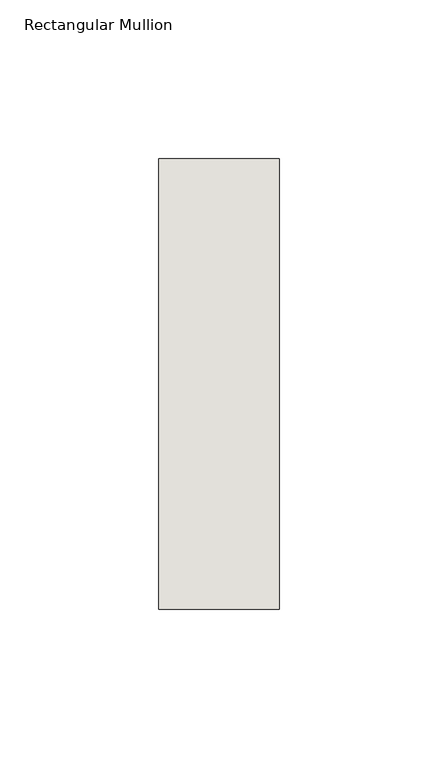
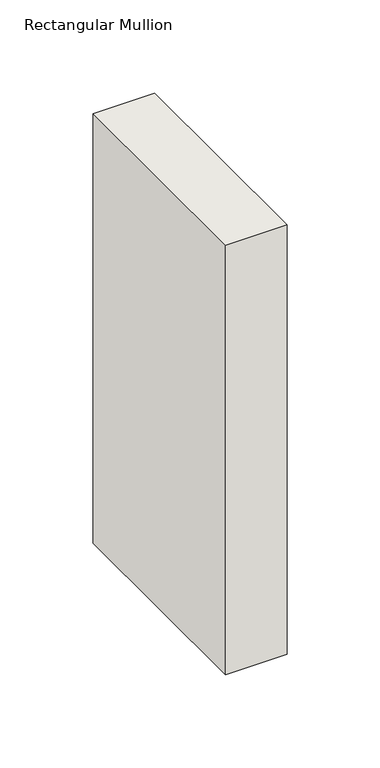
"""IFC4 building model written with IfcOpenShell, lengths in millimetres: wall geometry, Rectangular Mullion : NLRS_21_CWM_hsb-regel 38x142_gen_rsf."""

import ifcopenshell
import ifcopenshell.guid

model = None  # the IFC model being written
_history = None  # IfcOwnerHistory: only IFC2X3 demands one
_inside = {}  # id of a spatial element -> (the spatial element, [elements in it])
_under = {}  # id of a project, library or spatial element -> (it, [spatial elements below it])
_declared = {}  # id of a project -> (the project, [libraries it declares])
_typed = {}  # id of a type object -> (the type object, [elements of that type])
_made_of = {}  # id of a material, layer set ... -> (it, [elements and type objects made of it])


def new_model(schema):
    """Start an empty IFC model of exactly this schema.

    Asked for "IFC4X3", IfcOpenShell would pick the latest addendum, in which some entities
    have other attributes; the version numbers below select the first issue.
    IFC2X3 requires an IfcOwnerHistory on every rooted entity: one is made here for all.
    """
    global model, _history
    if schema == "IFC4X3":
        model = ifcopenshell.file(schema_version=(4, 3, 0, 0))
    else:
        model = ifcopenshell.file(schema=schema)
    _inside.clear()
    _under.clear()
    _declared.clear()
    _typed.clear()
    _made_of.clear()
    _history = None
    if model.schema == "IFC2X3":
        org = make("IfcOrganization", Name="unknown")
        user = make(
            "IfcPersonAndOrganization",
            ThePerson=make("IfcPerson", FamilyName="unknown"),
            TheOrganization=org,
        )
        app = make(
            "IfcApplication",
            ApplicationDeveloper=org,
            Version="unknown",
            ApplicationFullName="unknown",
            ApplicationIdentifier="unknown",
        )
        _history = make(
            "IfcOwnerHistory",
            OwningUser=user,
            OwningApplication=app,
            ChangeAction="ADDED",
            CreationDate=0,
        )
    return model


def make(cls, **values):
    """One entity of the class cls with the attributes given. An attribute that is None is left unset."""
    return model.create_entity(
        cls, **{name: value for name, value in values.items() if value is not None}
    )


def rooted(cls, **values):
    """An entity with a GlobalId (a new one), such as an element, a storey or a relation."""
    return make(cls, GlobalId=ifcopenshell.guid.new(), OwnerHistory=_history, **values)


def si_unit(unit_type, name, prefix=None):
    """IfcSIUnit, for example si_unit("LENGTHUNIT", "METRE", prefix="MILLI")."""
    return make("IfcSIUnit", UnitType=unit_type, Prefix=prefix, Name=name)


def assignment(units):
    """IfcUnitAssignment: the units of a project."""
    return None if units is None else make("IfcUnitAssignment", Units=units)


def point(xyz):
    """IfcCartesianPoint."""
    return None if xyz is None else make("IfcCartesianPoint", Coordinates=xyz)


def direction(xyz):
    """IfcDirection."""
    return None if xyz is None else make("IfcDirection", DirectionRatios=xyz)


def frame(location, z_axis=None, x_axis=None):
    """IfcAxis2Placement3D, a coordinate frame: its origin and axes. An axis left out is left unset."""
    return make(
        "IfcAxis2Placement3D",
        Location=point(location),
        Axis=direction(z_axis),
        RefDirection=direction(x_axis),
    )


def origin():
    """The frame at (0, 0, 0) with its axes left unset."""
    return frame((0.0, 0.0, 0.0))


def place(relative_to, where):
    """IfcLocalPlacement: puts the frame where relative to a parent placement (None: the world)."""
    return make(
        "IfcLocalPlacement", PlacementRelTo=relative_to, RelativePlacement=where
    )


def context(
    kind, dimensions, precision=None, world=None, true_north=None, identifier=None
):
    """IfcGeometricRepresentationContext, for example the 3D "Model" context."""
    return make(
        "IfcGeometricRepresentationContext",
        ContextIdentifier=identifier,
        ContextType=kind,
        CoordinateSpaceDimension=dimensions,
        Precision=precision,
        WorldCoordinateSystem=world,
        TrueNorth=true_north,
    )


def project(units=None, contexts=None):
    """IfcProject with its units and contexts."""
    return rooted(
        "IfcProject",
        Name="project",
        RepresentationContexts=contexts,
        UnitsInContext=assignment(units),
    )


def spatial(cls, under=None, at=None, **own):
    """A site, building, storey or space (cls), placed at a placement, below another one or the project."""
    s = rooted(cls, ObjectPlacement=at, **own)
    if under is not None:
        _under.setdefault(under.id(), (under, []))[1].append(s)
    return s


def polyline(points):
    """IfcPolyline through the points."""
    return make("IfcPolyline", Points=[point(p) for p in points])


def outline(outer, holes=None, kind="AREA"):
    """IfcArbitraryClosedProfileDef: a profile drawn as a closed curve; with holes, ...WithVoids."""
    if holes is None:
        return make("IfcArbitraryClosedProfileDef", ProfileType=kind, OuterCurve=outer)
    return make(
        "IfcArbitraryProfileDefWithVoids",
        ProfileType=kind,
        OuterCurve=outer,
        InnerCurves=holes,
    )


def extrude(swept, where, along, depth):
    """IfcExtrudedAreaSolid: the profile swept, set in the frame where, extruded along a direction by depth."""
    return make(
        "IfcExtrudedAreaSolid",
        SweptArea=swept,
        Position=where,
        ExtrudedDirection=direction(along),
        Depth=depth,
    )


def shape(context_of_items, identifier, shape_type, items):
    """IfcShapeRepresentation: the items that make up one representation, for example the "Body"."""
    return make(
        "IfcShapeRepresentation",
        ContextOfItems=context_of_items,
        RepresentationIdentifier=identifier,
        RepresentationType=shape_type,
        Items=items,
    )


def source(mapping_origin, context_of_items, identifier, shape_type, items):
    """IfcRepresentationMap: a shape defined once, which mapped items show again and again."""
    return make(
        "IfcRepresentationMap",
        MappingOrigin=mapping_origin,
        MappedRepresentation=shape(context_of_items, identifier, shape_type, items),
    )


def transform(
    local_origin,
    x_axis=None,
    y_axis=None,
    z_axis=None,
    scale=None,
    scale2=None,
    scale3=None,
    uniform=True,
):
    """IfcCartesianTransformationOperator3D, or its non-uniform kind. x_axis, y_axis, z_axis: its Axis1, 2, 3."""
    if uniform:
        return make(
            "IfcCartesianTransformationOperator3D",
            Axis1=direction(x_axis),
            Axis2=direction(y_axis),
            LocalOrigin=point(local_origin),
            Scale=scale,
            Axis3=direction(z_axis),
        )
    return make(
        "IfcCartesianTransformationOperator3DnonUniform",
        Axis1=direction(x_axis),
        Axis2=direction(y_axis),
        LocalOrigin=point(local_origin),
        Scale=scale,
        Axis3=direction(z_axis),
        Scale2=scale2,
        Scale3=scale3,
    )


def mapped(mapping_source, mapping_target):
    """IfcMappedItem: shows the shape of a source again, moved by a transform."""
    return make(
        "IfcMappedItem", MappingSource=mapping_source, MappingTarget=mapping_target
    )


def made_of(thing, what):
    """Note that an element or type object is made of a material, layer set ...; save() writes the relation."""
    if what is not None:
        _made_of.setdefault(what.id(), (what, []))[1].append(thing)
    return thing


def element(
    cls,
    number,
    at=None,
    inside=None,
    cuts=None,
    type_object=None,
    material=None,
    context=None,
    identifier="Body",
    shape_type=None,
    held_by="IfcProductDefinitionShape",
    body=None,
    shapes=None,
    **own,
):
    """One element of the class cls, such as IfcWall. Its Tag is "e" and its number.

    at: its placement. inside: the storey or other place that contains it. cuts: it is an
    opening in that element (IfcRelVoidsElement). A single representation is given by context,
    identifier, shape_type and body (its items); several are given by shapes. held_by: the class
    of the entity that holds the representations. save() writes the other relations.
    """
    e = rooted(cls, Tag="e%d" % number, ObjectPlacement=at, **own)
    if body is not None:
        shapes = [shape(context, identifier, shape_type, body)]
    if shapes is not None:
        e.Representation = make(held_by, Representations=shapes)
    if inside is not None:
        _inside.setdefault(inside.id(), (inside, []))[1].append(e)
    if cuts is not None:
        rooted(
            "IfcRelVoidsElement", RelatingBuildingElement=cuts, RelatedOpeningElement=e
        )
    if type_object is not None:
        _typed.setdefault(type_object.id(), (type_object, []))[1].append(e)
    return made_of(e, material)


def aggregate(whole, parts):
    """IfcRelAggregates: a whole, such as a stair, and the parts it consists of."""
    return rooted("IfcRelAggregates", RelatingObject=whole, RelatedObjects=parts)


def save(model, path):
    """Write the relations noted so far, then the file.

    IfcRelAggregates (storeys below a building ...), IfcRelContainedInSpatialStructure (elements
    in a storey), IfcRelDefinesByType, IfcRelAssociatesMaterial and IfcRelDeclares: one each for
    every whole, place, type object, material and project.
    """
    for whole, parts in _under.values():
        aggregate(whole, parts)
    for where, things in _inside.values():
        rooted(
            "IfcRelContainedInSpatialStructure",
            RelatedElements=things,
            RelatingStructure=where,
        )
    for kind, things in _typed.values():
        rooted("IfcRelDefinesByType", RelatedObjects=things, RelatingType=kind)
    for what, things in _made_of.values():
        rooted("IfcRelAssociatesMaterial", RelatedObjects=things, RelatingMaterial=what)
    for by, libraries in _declared.values():
        rooted("IfcRelDeclares", RelatingContext=by, RelatedDefinitions=libraries)
    model.write(path)


def rectangular_mullion_baa0df26(model_context):
    return source(origin(), model_context, "Body", "SweptSolid", [
        extrude(outline(polyline([(-38.0, -71.0), (-38.0, 71.0), (0.0, 71.0), (0.0, -71.0), (-38.0, -71.0)])), frame((0.0, 0.0, -280.9999997), z_axis=(0.0, 0.0, 1.0), x_axis=(1.0, 0.0, 0.0)), (0.0, 0.0, 1.0), 280.9999997),
    ])


if __name__ == "__main__":
    model = new_model("IFC4")
    model_context = context("Model", 3, world=origin())
    ifc_project = project(units=[si_unit("LENGTHUNIT", "METRE", prefix="MILLI")], contexts=[model_context])
    site = spatial("IfcSite", under=ifc_project)
    building = spatial("IfcBuilding", under=site)
    placement = place(None, origin())
    rectangular_mullion_shape = rectangular_mullion_baa0df26(model_context)
    element("IfcWall", 1, ObjectType="Rectangular Mullion : NLRS_21_CWM_hsb-regel 38x142_gen_rsf", at=placement, inside=building, context=model_context, shape_type="MappedRepresentation", body=[
        mapped(rectangular_mullion_shape, transform((0.0, 0.0, 0.0), x_axis=(1.0, 0.0, 0.0), y_axis=(0.0, 1.0, 0.0), z_axis=(0.0, 0.0, 1.0))),
    ])
    save(model, "model.ifc")

# Revit data of these elements
# Type "Rectangular Mullion : NLRS_21_CWM_hsb-regel 38x142_gen_rsf"
#   Type IfcGUID = "07M7mRoiH1CR8m_RSKIwpF"
#   Assembly Code = "21.10"
#   IfcExportAs = "IfcWall"
#   built-in parameter 1007322 = 0.465879 (stored number, unit not read)
#   built-in parameter 1007321 = 0.062336 (stored number, unit not read)
#   built-in parameter 1007320 = 0.062336 (stored number, unit not read)
# Element 1 (IfcWall, "Rectangular Mullion : NLRS_21_CWM_hsb-regel 38x142_gen_rsf")
#   Materials on its faces: "NLRS_i2_hout naaldhout vuren_gen_rsf"
# Materials
#   "NLRS_i2_hout naaldhout vuren_gen_rsf": class "I - Hout", colour RGB 234 199 147, transparency 0, Keynote = "i2", Manufacturer = "Revit Standards Foundation", URL = "www.revitstandards.org", Description = "hout vuren", Cost = 0
